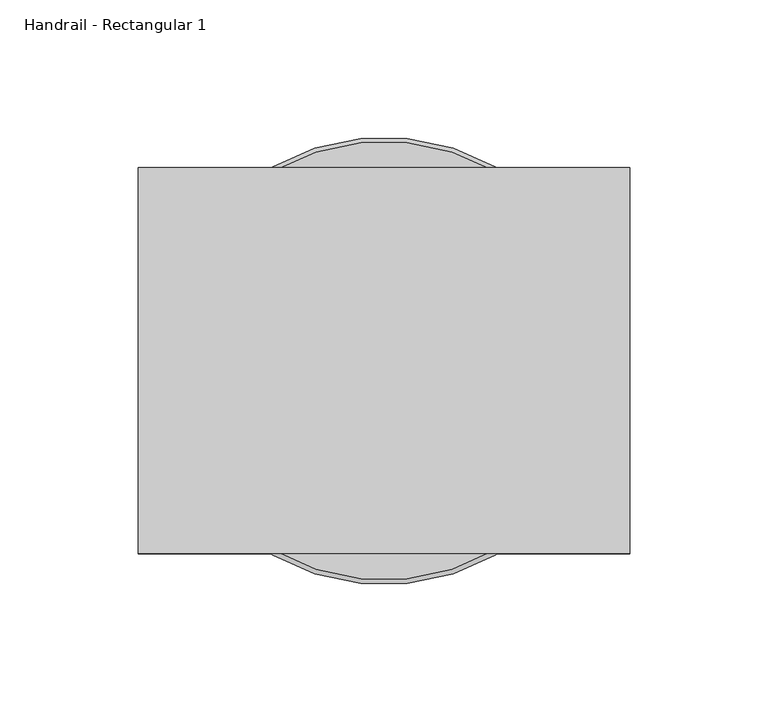
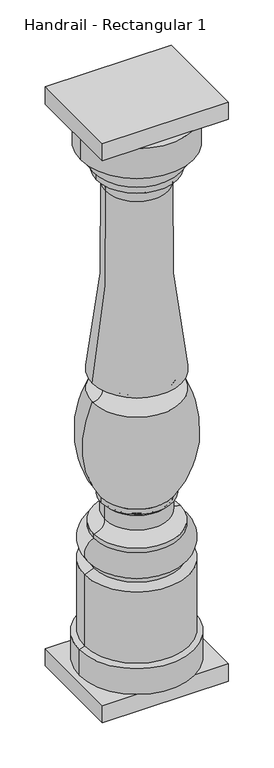
"""IFC4 building model written with IfcOpenShell, lengths in millimetres: railing geometry, Handrail - Rectangular 1."""

import ifcopenshell
import ifcopenshell.guid

model = None  # the IFC model being written
_history = None  # IfcOwnerHistory: only IFC2X3 demands one
_inside = {}  # id of a spatial element -> (the spatial element, [elements in it])
_under = {}  # id of a project, library or spatial element -> (it, [spatial elements below it])
_declared = {}  # id of a project -> (the project, [libraries it declares])
_typed = {}  # id of a type object -> (the type object, [elements of that type])
_made_of = {}  # id of a material, layer set ... -> (it, [elements and type objects made of it])


def new_model(schema):
    """Start an empty IFC model of exactly this schema.

    Asked for "IFC4X3", IfcOpenShell would pick the latest addendum, in which some entities
    have other attributes; the version numbers below select the first issue.
    IFC2X3 requires an IfcOwnerHistory on every rooted entity: one is made here for all.
    """
    global model, _history
    if schema == "IFC4X3":
        model = ifcopenshell.file(schema_version=(4, 3, 0, 0))
    else:
        model = ifcopenshell.file(schema=schema)
    _inside.clear()
    _under.clear()
    _declared.clear()
    _typed.clear()
    _made_of.clear()
    _history = None
    if model.schema == "IFC2X3":
        org = make("IfcOrganization", Name="unknown")
        user = make(
            "IfcPersonAndOrganization",
            ThePerson=make("IfcPerson", FamilyName="unknown"),
            TheOrganization=org,
        )
        app = make(
            "IfcApplication",
            ApplicationDeveloper=org,
            Version="unknown",
            ApplicationFullName="unknown",
            ApplicationIdentifier="unknown",
        )
        _history = make(
            "IfcOwnerHistory",
            OwningUser=user,
            OwningApplication=app,
            ChangeAction="ADDED",
            CreationDate=0,
        )
    return model


def make(cls, **values):
    """One entity of the class cls with the attributes given. An attribute that is None is left unset."""
    return model.create_entity(
        cls, **{name: value for name, value in values.items() if value is not None}
    )


def rooted(cls, **values):
    """An entity with a GlobalId (a new one), such as an element, a storey or a relation."""
    return make(cls, GlobalId=ifcopenshell.guid.new(), OwnerHistory=_history, **values)


def si_unit(unit_type, name, prefix=None):
    """IfcSIUnit, for example si_unit("LENGTHUNIT", "METRE", prefix="MILLI")."""
    return make("IfcSIUnit", UnitType=unit_type, Prefix=prefix, Name=name)


def assignment(units):
    """IfcUnitAssignment: the units of a project."""
    return None if units is None else make("IfcUnitAssignment", Units=units)


def point(xyz):
    """IfcCartesianPoint."""
    return None if xyz is None else make("IfcCartesianPoint", Coordinates=xyz)


def direction(xyz):
    """IfcDirection."""
    return None if xyz is None else make("IfcDirection", DirectionRatios=xyz)


def frame(location, z_axis=None, x_axis=None):
    """IfcAxis2Placement3D, a coordinate frame: its origin and axes. An axis left out is left unset."""
    return make(
        "IfcAxis2Placement3D",
        Location=point(location),
        Axis=direction(z_axis),
        RefDirection=direction(x_axis),
    )


def origin():
    """The frame at (0, 0, 0) with its axes left unset."""
    return frame((0.0, 0.0, 0.0))


def place(relative_to, where):
    """IfcLocalPlacement: puts the frame where relative to a parent placement (None: the world)."""
    return make(
        "IfcLocalPlacement", PlacementRelTo=relative_to, RelativePlacement=where
    )


def context(
    kind, dimensions, precision=None, world=None, true_north=None, identifier=None
):
    """IfcGeometricRepresentationContext, for example the 3D "Model" context."""
    return make(
        "IfcGeometricRepresentationContext",
        ContextIdentifier=identifier,
        ContextType=kind,
        CoordinateSpaceDimension=dimensions,
        Precision=precision,
        WorldCoordinateSystem=world,
        TrueNorth=true_north,
    )


def project(units=None, contexts=None):
    """IfcProject with its units and contexts."""
    return rooted(
        "IfcProject",
        Name="project",
        RepresentationContexts=contexts,
        UnitsInContext=assignment(units),
    )


def spatial(cls, under=None, at=None, **own):
    """A site, building, storey or space (cls), placed at a placement, below another one or the project."""
    s = rooted(cls, ObjectPlacement=at, **own)
    if under is not None:
        _under.setdefault(under.id(), (under, []))[1].append(s)
    return s


def polyline(points):
    """IfcPolyline through the points."""
    return make("IfcPolyline", Points=[point(p) for p in points])


def circle_curve(where, radius):
    """IfcCircle in the frame where."""
    return make("IfcCircle", Position=where, Radius=radius)


def ellipse_curve(where, semi_axis1, semi_axis2):
    """IfcEllipse in the frame where."""
    return make(
        "IfcEllipse", Position=where, SemiAxis1=semi_axis1, SemiAxis2=semi_axis2
    )


def trimmed(basis, trim1, trim2, sense, master):
    """IfcTrimmedCurve: the piece of a basis curve between two trims."""
    return make(
        "IfcTrimmedCurve",
        BasisCurve=basis,
        Trim1=trim1,
        Trim2=trim2,
        SenseAgreement=sense,
        MasterRepresentation=master,
    )


def outline(outer, holes=None, kind="AREA"):
    """IfcArbitraryClosedProfileDef: a profile drawn as a closed curve; with holes, ...WithVoids."""
    if holes is None:
        return make("IfcArbitraryClosedProfileDef", ProfileType=kind, OuterCurve=outer)
    return make(
        "IfcArbitraryProfileDefWithVoids",
        ProfileType=kind,
        OuterCurve=outer,
        InnerCurves=holes,
    )


def extrude(swept, where, along, depth):
    """IfcExtrudedAreaSolid: the profile swept, set in the frame where, extruded along a direction by depth."""
    return make(
        "IfcExtrudedAreaSolid",
        SweptArea=swept,
        Position=where,
        ExtrudedDirection=direction(along),
        Depth=depth,
    )


def shape(context_of_items, identifier, shape_type, items):
    """IfcShapeRepresentation: the items that make up one representation, for example the "Body"."""
    return make(
        "IfcShapeRepresentation",
        ContextOfItems=context_of_items,
        RepresentationIdentifier=identifier,
        RepresentationType=shape_type,
        Items=items,
    )


def source(mapping_origin, context_of_items, identifier, shape_type, items):
    """IfcRepresentationMap: a shape defined once, which mapped items show again and again."""
    return make(
        "IfcRepresentationMap",
        MappingOrigin=mapping_origin,
        MappedRepresentation=shape(context_of_items, identifier, shape_type, items),
    )


def transform(
    local_origin,
    x_axis=None,
    y_axis=None,
    z_axis=None,
    scale=None,
    scale2=None,
    scale3=None,
    uniform=True,
):
    """IfcCartesianTransformationOperator3D, or its non-uniform kind. x_axis, y_axis, z_axis: its Axis1, 2, 3."""
    if uniform:
        return make(
            "IfcCartesianTransformationOperator3D",
            Axis1=direction(x_axis),
            Axis2=direction(y_axis),
            LocalOrigin=point(local_origin),
            Scale=scale,
            Axis3=direction(z_axis),
        )
    return make(
        "IfcCartesianTransformationOperator3DnonUniform",
        Axis1=direction(x_axis),
        Axis2=direction(y_axis),
        LocalOrigin=point(local_origin),
        Scale=scale,
        Axis3=direction(z_axis),
        Scale2=scale2,
        Scale3=scale3,
    )


def mapped(mapping_source, mapping_target):
    """IfcMappedItem: shows the shape of a source again, moved by a transform."""
    return make(
        "IfcMappedItem", MappingSource=mapping_source, MappingTarget=mapping_target
    )


def made_of(thing, what):
    """Note that an element or type object is made of a material, layer set ...; save() writes the relation."""
    if what is not None:
        _made_of.setdefault(what.id(), (what, []))[1].append(thing)
    return thing


def element(
    cls,
    number,
    at=None,
    inside=None,
    cuts=None,
    type_object=None,
    material=None,
    context=None,
    identifier="Body",
    shape_type=None,
    held_by="IfcProductDefinitionShape",
    body=None,
    shapes=None,
    **own,
):
    """One element of the class cls, such as IfcWall. Its Tag is "e" and its number.

    at: its placement. inside: the storey or other place that contains it. cuts: it is an
    opening in that element (IfcRelVoidsElement). A single representation is given by context,
    identifier, shape_type and body (its items); several are given by shapes. held_by: the class
    of the entity that holds the representations. save() writes the other relations.
    """
    e = rooted(cls, Tag="e%d" % number, ObjectPlacement=at, **own)
    if body is not None:
        shapes = [shape(context, identifier, shape_type, body)]
    if shapes is not None:
        e.Representation = make(held_by, Representations=shapes)
    if inside is not None:
        _inside.setdefault(inside.id(), (inside, []))[1].append(e)
    if cuts is not None:
        rooted(
            "IfcRelVoidsElement", RelatingBuildingElement=cuts, RelatedOpeningElement=e
        )
    if type_object is not None:
        _typed.setdefault(type_object.id(), (type_object, []))[1].append(e)
    return made_of(e, material)


def aggregate(whole, parts):
    """IfcRelAggregates: a whole, such as a stair, and the parts it consists of."""
    return rooted("IfcRelAggregates", RelatingObject=whole, RelatedObjects=parts)


def save(model, path):
    """Write the relations noted so far, then the file.

    IfcRelAggregates (storeys below a building ...), IfcRelContainedInSpatialStructure (elements
    in a storey), IfcRelDefinesByType, IfcRelAssociatesMaterial and IfcRelDeclares: one each for
    every whole, place, type object, material and project.
    """
    for whole, parts in _under.values():
        aggregate(whole, parts)
    for where, things in _inside.values():
        rooted(
            "IfcRelContainedInSpatialStructure",
            RelatedElements=things,
            RelatingStructure=where,
        )
    for kind, things in _typed.values():
        rooted("IfcRelDefinesByType", RelatedObjects=things, RelatingType=kind)
    for what, things in _made_of.values():
        rooted("IfcRelAssociatesMaterial", RelatedObjects=things, RelatingMaterial=what)
    for by, libraries in _declared.values():
        rooted("IfcRelDeclares", RelatingContext=by, RelatedDefinitions=libraries)
    model.write(path)


def plane_surface(at):
    """IfcPlane: the flat surface through the origin of the frame at, square to its z axis."""
    return make("IfcPlane", Position=at)


def cylinder_surface(at, radius):
    """IfcCylindricalSurface: all points at the distance radius from the z axis of the frame at."""
    return make("IfcCylindricalSurface", Position=at, Radius=radius)


def revolved_surface(curve, axis_point, axis_direction):
    """IfcSurfaceOfRevolution: the curve turned about the line through axis_point along axis_direction."""
    return make(
        "IfcSurfaceOfRevolution",
        SweptCurve=make("IfcArbitraryOpenProfileDef", ProfileType="CURVE", Curve=curve),
        AxisPosition=make("IfcAxis1Placement", Location=point(axis_point), Axis=direction(axis_direction)),
    )


def advanced_brep(points, edges, surfaces, faces):
    """IfcAdvancedBrep: a solid bounded by faces that lie on surfaces and meet in shared edges.

    An edge is (start, end): straight between two places in points (the first is 0);
    or (start, end, curve); or (start, end, curve, False) where it runs against its curve.
    A face is (place in surfaces, loops), or (place, loops, False) where it looks against
    its surface's normal. A loop lists edges by number (the first is 1), with a minus sign
    where the edge is run from its end to its start. The first loop is the outer one.
    """
    corners = [point(p) for p in points]
    vertices = [make("IfcVertexPoint", VertexGeometry=c) for c in corners]
    made = []
    for start, end, *more in edges:
        made.append(
            make(
                "IfcEdgeCurve",
                EdgeStart=vertices[start],
                EdgeEnd=vertices[end],
                EdgeGeometry=more[0] if more else make("IfcPolyline", Points=[corners[start], corners[end]]),
                SameSense=more[1] if len(more) > 1 else True,
            )
        )
    hull = []
    for where, loops, *sense in faces:
        bounds = []
        for j, loop in enumerate(loops):
            ring = [make("IfcOrientedEdge", EdgeElement=made[abs(k) - 1], Orientation=k > 0) for k in loop]
            bounds.append(
                make(
                    "IfcFaceOuterBound" if j == 0 else "IfcFaceBound",
                    Bound=make("IfcEdgeLoop", EdgeList=ring),
                    Orientation=True,
                )
            )
        hull.append(make("IfcAdvancedFace", Bounds=bounds, FaceSurface=surfaces[where], SameSense=sense[0] if sense else True))
    return make("IfcAdvancedBrep", Outer=make("IfcClosedShell", CfsFaces=hull))


def handrail_rectangular_1_85a9581f(model_context):
    return source(origin(), model_context, "Body", "SolidModel", [
        advanced_brep(
        [(6614.0521895, -1665.6164768, 939.8), (6534.6771895, -1665.6164768, 939.8), (6693.4271895, -1665.6164768, 939.8), (6695.0146895, -1665.6164768, 127.0), (6533.0896895, -1665.6164768, 127.0), (6614.0521895, -1665.6164768, 127.0), (6695.0146895, -1665.6164768, 165.2785542), (6533.0896895, -1665.6164768, 165.2785542), (6687.8709395, -1665.6164768, 168.275), (6540.2334395, -1665.6164768, 168.275), (6687.8709395, -1665.6164768, 274.7335284), (6540.2334395, -1665.6164768, 274.7335284), (6675.1709395, -1665.6164768, 280.19375), (6552.9334395, -1665.6164768, 280.19375), (6675.1709395, -1665.6164768, 286.54375), (6552.9334395, -1665.6164768, 286.54375), (6675.1709395, -1665.6164768, 324.64375), (6552.9334395, -1665.6164768, 324.64375), (6675.1709395, -1665.6164768, 330.99375), (6552.9334395, -1665.6164768, 330.99375), (6659.4640435, -1665.6164768, 347.276159), (6568.6403356, -1665.6164768, 347.276159), (6659.4640435, -1665.6164768, 368.8906259), (6568.6403356, -1665.6164768, 368.8906259), (6664.0584395, -1665.6164768, 373.85625), (6564.0459395, -1665.6164768, 373.85625), (6664.0584395, -1665.6164768, 381.4842759), (6564.0459395, -1665.6164768, 381.4842759), (6676.7584395, -1665.6164768, 527.84375), (6551.3459395, -1665.6164768, 527.84375), (6676.7584395, -1665.6164768, 556.41875), (6551.3459395, -1665.6164768, 556.41875), (6658.2243377, -1665.6164768, 836.1713606), (6569.8800414, -1665.6164768, 836.1713606), (6671.2021895, -1665.6164768, 858.04375), (6556.9021895, -1665.6164768, 858.04375), (6671.2021895, -1665.6164768, 866.775), (6556.9021895, -1665.6164768, 866.775), (6682.3146895, -1665.6164768, 892.175), (6545.7896895, -1665.6164768, 892.175), (6693.4271895, -1665.6164768, 895.35), (6534.6771895, -1665.6164768, 895.35)],
        [
            (0, 1),
            (1, 2, circle_curve(frame((6614.0521895, -1665.6164768, 939.8), z_axis=(0.0, 0.0, 1.0), x_axis=(-1.0, 0.0, 0.0)), 79.375)),
            (2, 0),
            (2, 1, circle_curve(frame((6614.0521895, -1665.6164768, 939.8), z_axis=(0.0, 0.0, 1.0), x_axis=(-1.0, 0.0, 0.0)), 79.375)),
            (3, 4, circle_curve(frame((6614.0521895, -1665.6164768, 127.0), z_axis=(0.0, 0.0, -1.0), x_axis=(-1.0, 0.0, 0.0)), 80.9625)),
            (4, 5),
            (5, 3),
            (4, 3, circle_curve(frame((6614.0521895, -1665.6164768, 127.0), z_axis=(0.0, 0.0, -1.0), x_axis=(-1.0, 0.0, 0.0)), 80.9625)),
            (6, 7, circle_curve(frame((6614.0521895, -1665.6164768, 165.2785542), z_axis=(0.0, 0.0, -1.0), x_axis=(-1.0, 0.0, 0.0)), 80.9625)),
            (7, 4),
            (3, 6),
            (7, 6, circle_curve(frame((6614.0521895, -1665.6164768, 165.2785542), z_axis=(0.0, 0.0, -1.0), x_axis=(-1.0, 0.0, 0.0)), 80.9625)),
            (8, 9, circle_curve(frame((6614.0521895, -1665.6164768, 168.275), z_axis=(0.0, 0.0, -1.0), x_axis=(-1.0, 0.0, 0.0)), 73.81875)),
            (9, 7),
            (6, 8),
            (9, 8, circle_curve(frame((6614.0521895, -1665.6164768, 168.275), z_axis=(0.0, 0.0, -1.0), x_axis=(-1.0, 0.0, 0.0)), 73.81875)),
            (10, 11, circle_curve(frame((6614.0521895, -1665.6164768, 274.7335284), z_axis=(0.0, 0.0, -1.0), x_axis=(-1.0, 0.0, 0.0)), 73.81875)),
            (11, 9),
            (8, 10),
            (11, 10, circle_curve(frame((6614.0521895, -1665.6164768, 274.7335284), z_axis=(0.0, 0.0, -1.0), x_axis=(-1.0, 0.0, 0.0)), 73.81875)),
            (12, 13, circle_curve(frame((6614.0521895, -1665.6164768, 280.19375), z_axis=(0.0, 0.0, -1.0), x_axis=(-1.0, 0.0, 0.0)), 61.11875)),
            (13, 11),
            (10, 12),
            (13, 12, circle_curve(frame((6614.0521895, -1665.6164768, 280.19375), z_axis=(0.0, 0.0, -1.0), x_axis=(-1.0, 0.0, 0.0)), 61.11875)),
            (14, 15, circle_curve(frame((6614.0521895, -1665.6164768, 286.54375), z_axis=(0.0, 0.0, -1.0), x_axis=(-1.0, 0.0, 0.0)), 61.11875)),
            (15, 13),
            (12, 14),
            (15, 14, circle_curve(frame((6614.0521895, -1665.6164768, 286.54375), z_axis=(0.0, 0.0, -1.0), x_axis=(-1.0, 0.0, 0.0)), 61.11875)),
            (16, 17, circle_curve(frame((6614.0521895, -1665.6164768, 324.64375), z_axis=(0.0, 0.0, -1.0), x_axis=(-1.0, 0.0, 0.0)), 61.11875)),
            (17, 15, circle_curve(frame((6561.1987498, -1665.6164768, 305.59375), z_axis=(0.0, -1.0, 0.0), x_axis=(1.0, 0.0, 0.0)), 20.7657856)),
            (14, 16, circle_curve(frame((6666.9056293, -1665.6164768, 305.59375), z_axis=(0.0, -1.0, 0.0), x_axis=(-1.0, 0.0, 0.0)), 20.7657856)),
            (17, 16, circle_curve(frame((6614.0521895, -1665.6164768, 324.64375), z_axis=(0.0, 0.0, -1.0), x_axis=(-1.0, 0.0, 0.0)), 61.11875)),
            (18, 19, circle_curve(frame((6614.0521895, -1665.6164768, 330.99375), z_axis=(0.0, 0.0, -1.0), x_axis=(-1.0, 0.0, 0.0)), 61.11875)),
            (19, 17),
            (16, 18),
            (19, 18, circle_curve(frame((6614.0521895, -1665.6164768, 330.99375), z_axis=(0.0, 0.0, -1.0), x_axis=(-1.0, 0.0, 0.0)), 61.11875)),
            (20, 21, circle_curve(frame((6614.0521895, -1665.6164768, 347.276159), z_axis=(0.0, 0.0, -1.0), x_axis=(-1.0, 0.0, 0.0)), 45.4118539)),
            (21, 19, circle_curve(frame((6553.4004121, -1665.6164768, 346.26035), z_axis=(0.0, 1.0, 0.0), x_axis=(1.0, 0.0, 0.0)), 15.2737402)),
            (18, 20, circle_curve(frame((6674.703967, -1665.6164768, 346.26035), z_axis=(0.0, 1.0, 0.0), x_axis=(-1.0, 0.0, 0.0)), 15.2737402)),
            (21, 20, circle_curve(frame((6614.0521895, -1665.6164768, 347.276159), z_axis=(0.0, 0.0, -1.0), x_axis=(-1.0, 0.0, 0.0)), 45.4118539)),
            (22, 23, circle_curve(frame((6614.0521895, -1665.6164768, 368.8906259), z_axis=(0.0, 0.0, -1.0), x_axis=(-1.0, 0.0, 0.0)), 45.4118539)),
            (23, 21),
            (20, 22),
            (23, 22, circle_curve(frame((6614.0521895, -1665.6164768, 368.8906259), z_axis=(0.0, 0.0, -1.0), x_axis=(-1.0, 0.0, 0.0)), 45.4118539)),
            (24, 25, circle_curve(frame((6614.0521895, -1665.6164768, 373.85625), z_axis=(0.0, 0.0, -1.0), x_axis=(-1.0, 0.0, 0.0)), 50.00625)),
            (25, 23, circle_curve(frame((6563.7940931, -1665.6164768, 369.014959), z_axis=(0.0, 1.0, 0.0), x_axis=(1.0, 0.0, 0.0)), 4.8478372)),
            (22, 24, circle_curve(frame((6664.310286, -1665.6164768, 369.014959), z_axis=(0.0, 1.0, 0.0), x_axis=(-1.0, 0.0, 0.0)), 4.8478372)),
            (25, 24, circle_curve(frame((6614.0521895, -1665.6164768, 373.85625), z_axis=(0.0, 0.0, -1.0), x_axis=(-1.0, 0.0, 0.0)), 50.00625)),
            (26, 27, circle_curve(frame((6614.0521895, -1665.6164768, 381.4842759), z_axis=(0.0, 0.0, -1.0), x_axis=(-1.0, 0.0, 0.0)), 50.00625)),
            (27, 25),
            (24, 26),
            (27, 26, circle_curve(frame((6614.0521895, -1665.6164768, 381.4842759), z_axis=(0.0, 0.0, -1.0), x_axis=(-1.0, 0.0, 0.0)), 50.00625)),
            (28, 29, circle_curve(frame((6614.0521895, -1665.6164768, 527.84375), z_axis=(0.0, 0.0, -1.0), x_axis=(-1.0, 0.0, 0.0)), 62.70625)),
            (29, 27, circle_curve(frame((6681.6829206, -1665.6164768, 465.4226923), z_axis=(0.0, -1.0, 0.0), x_axis=(1.0, 0.0, 0.0)), 144.5133802)),
            (26, 28, circle_curve(frame((6546.4214585, -1665.6164768, 465.4226923), z_axis=(0.0, -1.0, 0.0), x_axis=(-1.0, 0.0, 0.0)), 144.5133802)),
            (29, 28, circle_curve(frame((6614.0521895, -1665.6164768, 527.84375), z_axis=(0.0, 0.0, -1.0), x_axis=(-1.0, 0.0, 0.0)), 62.70625)),
            (30, 31, circle_curve(frame((6614.0521895, -1665.6164768, 556.41875), z_axis=(0.0, 0.0, -1.0), x_axis=(-1.0, 0.0, 0.0)), 62.70625)),
            (31, 29, circle_curve(frame((6552.1940628, -1665.6164768, 542.13125), z_axis=(0.0, 1.0, 0.0), x_axis=(1.0, 0.0, 0.0)), 14.3126507)),
            (28, 30, circle_curve(frame((6675.9103163, -1665.6164768, 542.13125), z_axis=(0.0, 1.0, 0.0), x_axis=(-1.0, 0.0, 0.0)), 14.3126507)),
            (31, 30, circle_curve(frame((6614.0521895, -1665.6164768, 556.41875), z_axis=(0.0, 0.0, -1.0), x_axis=(-1.0, 0.0, 0.0)), 62.70625)),
            (32, 33, circle_curve(frame((6614.0521895, -1665.6164768, 836.1713606), z_axis=(0.0, 0.0, -1.0), x_axis=(-1.0, 0.0, 0.0)), 44.1721482)),
            (33, 31, circle_curve(frame((5440.060691, -1665.6164768, 770.5336134), z_axis=(0.0, 1.0, 0.0), x_axis=(1.0, 0.0, 0.0)), 1131.7243827)),
            (30, 32, circle_curve(frame((7788.0436881, -1665.6164768, 770.5336134), z_axis=(0.0, 1.0, 0.0), x_axis=(-1.0, 0.0, 0.0)), 1131.7243827)),
            (33, 32, circle_curve(frame((6614.0521895, -1665.6164768, 836.1713606), z_axis=(0.0, 0.0, -1.0), x_axis=(-1.0, 0.0, 0.0)), 44.1721482)),
            (34, 35, circle_curve(frame((6614.0521895, -1665.6164768, 858.04375), z_axis=(0.0, 0.0, -1.0), x_axis=(-1.0, 0.0, 0.0)), 57.15)),
            (35, 33, circle_curve(frame((6548.8577367, -1665.6164768, 838.4842616), z_axis=(0.0, 1.0, 0.0), x_axis=(1.0, 0.0, 0.0)), 21.1491562)),
            (32, 34, circle_curve(frame((6679.2466424, -1665.6164768, 838.4842616), z_axis=(0.0, 1.0, 0.0), x_axis=(-1.0, 0.0, 0.0)), 21.1491562)),
            (35, 34, circle_curve(frame((6614.0521895, -1665.6164768, 858.04375), z_axis=(0.0, 0.0, -1.0), x_axis=(-1.0, 0.0, 0.0)), 57.15)),
            (36, 37, circle_curve(frame((6614.0521895, -1665.6164768, 866.775), z_axis=(0.0, 0.0, -1.0), x_axis=(-1.0, 0.0, 0.0)), 57.15)),
            (37, 35),
            (34, 36),
            (37, 36, circle_curve(frame((6614.0521895, -1665.6164768, 866.775), z_axis=(0.0, 0.0, -1.0), x_axis=(-1.0, 0.0, 0.0)), 57.15)),
            (38, 39, circle_curve(frame((6614.0521895, -1665.6164768, 892.175), z_axis=(0.0, 0.0, -1.0), x_axis=(-1.0, 0.0, 0.0)), 68.2625)),
            (39, 37, circle_curve(frame((6575.1272944, -1665.6164768, 889.8793427), z_axis=(0.0, -1.0, 0.0), x_axis=(1.0, 0.0, 0.0)), 29.4272849)),
            (36, 38, circle_curve(frame((6652.9770847, -1665.6164768, 889.8793427), z_axis=(0.0, -1.0, 0.0), x_axis=(-1.0, 0.0, 0.0)), 29.4272849)),
            (39, 38, circle_curve(frame((6614.0521895, -1665.6164768, 892.175), z_axis=(0.0, 0.0, -1.0), x_axis=(-1.0, 0.0, 0.0)), 68.2625)),
            (40, 41, circle_curve(frame((6614.0521895, -1665.6164768, 895.35), z_axis=(0.0, 0.0, -1.0), x_axis=(-1.0, 0.0, 0.0)), 79.375)),
            (41, 39),
            (38, 40),
            (41, 40, circle_curve(frame((6614.0521895, -1665.6164768, 895.35), z_axis=(0.0, 0.0, -1.0), x_axis=(-1.0, 0.0, 0.0)), 79.375)),
            (1, 41),
            (40, 2),
        ],
        [
            plane_surface(frame((6614.0521895, -1665.6164768, 939.8), z_axis=(0.0, 0.0, 1.0), x_axis=(-1.0, 0.0, 0.0))),
            plane_surface(frame((6614.0521895, -1665.6164768, 127.0), z_axis=(0.0, 0.0, -1.0), x_axis=(-1.0, 0.0, 0.0))),
            cylinder_surface(frame((6614.0521895, -1665.6164768, 1009.65), z_axis=(0.0, 0.0, 1.0), x_axis=(-1.0, 0.0, 0.0)), 80.9625),
            revolved_surface(polyline([(6533.0896895, -1665.6164768, 165.2785542), (6540.2334395, -1665.6164768, 168.275)]), (6614.0521895, -1665.6164768, 1009.65), (0.0, 0.0, 1.0)),
            cylinder_surface(frame((6614.0521895, -1665.6164768, 1009.65), z_axis=(0.0, 0.0, 1.0), x_axis=(-1.0, 0.0, 0.0)), 73.81875),
            revolved_surface(polyline([(6540.2334395, -1665.6164768, 274.7335284), (6552.9334395, -1665.6164768, 280.19375)]), (6614.0521895, -1665.6164768, 1009.65), (0.0, 0.0, 1.0)),
            cylinder_surface(frame((6614.0521895, -1665.6164768, 1009.65), z_axis=(0.0, 0.0, 1.0), x_axis=(-1.0, 0.0, 0.0)), 61.11875),
            revolved_surface(trimmed(ellipse_curve(frame((6561.1987498, -1665.6164768, 305.59375), z_axis=(0.0, 1.0, 0.0), x_axis=(1.0, 0.0, 0.0)), 20.7657856, 20.7657856), [point((6552.9334395, -1665.6164768, 286.54375))], [point((6552.9334395, -1665.6164768, 324.64375))], True, "CARTESIAN"), (6614.0521895, -1665.6164768, 1009.65), (0.0, 0.0, 1.0)),
            revolved_surface(trimmed(ellipse_curve(frame((6553.4004121, -1665.6164768, 346.26035), z_axis=(0.0, -1.0, 0.0), x_axis=(1.0, 0.0, 0.0)), 15.2737402, 15.2737402), [point((6552.9334395, -1665.6164768, 330.99375))], [point((6568.6403356, -1665.6164768, 347.276159))], True, "CARTESIAN"), (6614.0521895, -1665.6164768, 1009.65), (0.0, 0.0, 1.0)),
            cylinder_surface(frame((6614.0521895, -1665.6164768, 1009.65), z_axis=(0.0, 0.0, 1.0), x_axis=(-1.0, 0.0, 0.0)), 45.4118539),
            revolved_surface(trimmed(ellipse_curve(frame((6563.7940931, -1665.6164768, 369.014959), z_axis=(0.0, -1.0, 0.0), x_axis=(1.0, 0.0, 0.0)), 4.8478372, 4.8478372), [point((6568.6403356, -1665.6164768, 368.8906259))], [point((6564.0459395, -1665.6164768, 373.85625))], True, "CARTESIAN"), (6614.0521895, -1665.6164768, 1009.65), (0.0, 0.0, 1.0)),
            cylinder_surface(frame((6614.0521895, -1665.6164768, 1009.65), z_axis=(0.0, 0.0, 1.0), x_axis=(-1.0, 0.0, 0.0)), 50.00625),
            revolved_surface(trimmed(ellipse_curve(frame((6681.6829206, -1665.6164768, 465.4226923), z_axis=(0.0, 1.0, 0.0), x_axis=(1.0, 0.0, 0.0)), 144.5133802, 144.5133802), [point((6564.0459395, -1665.6164768, 381.4842759))], [point((6551.3459395, -1665.6164768, 527.84375))], True, "CARTESIAN"), (6614.0521895, -1665.6164768, 1009.65), (0.0, 0.0, 1.0)),
            revolved_surface(trimmed(ellipse_curve(frame((6552.1940628, -1665.6164768, 542.13125), z_axis=(0.0, -1.0, 0.0), x_axis=(1.0, 0.0, 0.0)), 14.3126507, 14.3126507), [point((6551.3459395, -1665.6164768, 527.84375))], [point((6551.3459395, -1665.6164768, 556.41875))], True, "CARTESIAN"), (6614.0521895, -1665.6164768, 1009.65), (0.0, 0.0, 1.0)),
            revolved_surface(trimmed(ellipse_curve(frame((5440.060691, -1665.6164768, 770.5336134), z_axis=(0.0, -1.0, 0.0), x_axis=(1.0, 0.0, 0.0)), 1131.7243827, 1131.7243827), [point((6551.3459395, -1665.6164768, 556.41875))], [point((6569.8800414, -1665.6164768, 836.1713606))], True, "CARTESIAN"), (6614.0521895, -1665.6164768, 1009.65), (0.0, 0.0, 1.0)),
            revolved_surface(trimmed(ellipse_curve(frame((6548.8577367, -1665.6164768, 838.4842616), z_axis=(0.0, -1.0, 0.0), x_axis=(1.0, 0.0, 0.0)), 21.1491562, 21.1491562), [point((6569.8800414, -1665.6164768, 836.1713606))], [point((6556.9021895, -1665.6164768, 858.04375))], True, "CARTESIAN"), (6614.0521895, -1665.6164768, 1009.65), (0.0, 0.0, 1.0)),
            cylinder_surface(frame((6614.0521895, -1665.6164768, 1009.65), z_axis=(0.0, 0.0, 1.0), x_axis=(-1.0, 0.0, 0.0)), 57.15),
            revolved_surface(trimmed(ellipse_curve(frame((6575.1272944, -1665.6164768, 889.8793427), z_axis=(0.0, 1.0, 0.0), x_axis=(1.0, 0.0, 0.0)), 29.4272849, 29.4272849), [point((6556.9021895, -1665.6164768, 866.775))], [point((6545.7896895, -1665.6164768, 892.175))], True, "CARTESIAN"), (6614.0521895, -1665.6164768, 1009.65), (0.0, 0.0, 1.0)),
            revolved_surface(polyline([(6545.7896895, -1665.6164768, 892.175), (6534.6771895, -1665.6164768, 895.35)]), (6614.0521895, -1665.6164768, 1009.65), (0.0, 0.0, 1.0)),
            cylinder_surface(frame((6614.0521895, -1665.6164768, 1009.65), z_axis=(0.0, 0.0, 1.0), x_axis=(-1.0, 0.0, 0.0)), 79.375),
        ],
        [
            (0, [[1, 2, 3]]),
            (0, [[-3, 4, -1]]),
            (1, [[5, 6, 7]]),
            (1, [[8, -7, -6]]),
            (2, [[9, 10, -5, 11]]),
            (2, [[12, -11, -8, -10]]),
            (3, [[13, 14, -9, 15]]),
            (3, [[16, -15, -12, -14]]),
            (4, [[17, 18, -13, 19]]),
            (4, [[20, -19, -16, -18]]),
            (5, [[21, 22, -17, 23]]),
            (5, [[24, -23, -20, -22]]),
            (6, [[25, 26, -21, 27]]),
            (6, [[28, -27, -24, -26]]),
            (7, [[29, 30, -25, 31]]),
            (7, [[32, -31, -28, -30]]),
            (6, [[33, 34, -29, 35]]),
            (6, [[36, -35, -32, -34]]),
            (8, [[37, 38, -33, 39]]),
            (8, [[40, -39, -36, -38]]),
            (9, [[41, 42, -37, 43]]),
            (9, [[44, -43, -40, -42]]),
            (10, [[45, 46, -41, 47]]),
            (10, [[48, -47, -44, -46]]),
            (11, [[49, 50, -45, 51]]),
            (11, [[52, -51, -48, -50]]),
            (12, [[53, 54, -49, 55]]),
            (12, [[56, -55, -52, -54]]),
            (13, [[57, 58, -53, 59]]),
            (13, [[60, -59, -56, -58]]),
            (14, [[61, 62, -57, 63]]),
            (14, [[64, -63, -60, -62]]),
            (15, [[65, 66, -61, 67]]),
            (15, [[68, -67, -64, -66]]),
            (16, [[69, 70, -65, 71]]),
            (16, [[72, -71, -68, -70]]),
            (17, [[73, 74, -69, 75]]),
            (17, [[76, -75, -72, -74]]),
            (18, [[77, 78, -73, 79]]),
            (18, [[80, -79, -76, -78]]),
            (19, [[-2, 81, -77, 82]]),
            (19, [[-4, -82, -80, -81]]),
        ],
    ),
        extrude(outline(polyline([(6525.1521895, -1735.4664768), (6525.1521895, -1595.7664768), (6702.9521895, -1595.7664768), (6702.9521895, -1735.4664768), (6525.1521895, -1735.4664768)])), frame((0.0, 0.0, 101.6), z_axis=(0.0, 0.0, 1.0), x_axis=(1.0, 0.0, 0.0)), (0.0, 0.0, 1.0), 25.4),
        extrude(outline(polyline([(6525.1521895, -1595.7664768), (6702.9521895, -1595.7664768), (6702.9521895, -1735.4664768), (6525.1521895, -1735.4664768), (6525.1521895, -1595.7664768)])), frame((0.0, 0.0, 939.8), z_axis=(0.0, 0.0, 1.0), x_axis=(1.0, 0.0, 0.0)), (0.0, 0.0, 1.0), 25.4),
    ])


if __name__ == "__main__":
    model = new_model("IFC4")
    model_context = context("Model", 3, world=origin())
    ifc_project = project(units=[si_unit("LENGTHUNIT", "METRE", prefix="MILLI")], contexts=[model_context])
    site = spatial("IfcSite", under=ifc_project)
    building = spatial("IfcBuilding", under=site)
    placement = place(None, origin())
    handrail_rectangular_1_shape = handrail_rectangular_1_85a9581f(model_context)
    element("IfcRailing", 1, ObjectType="Handrail - Rectangular 1", at=placement, inside=building, context=model_context, shape_type="MappedRepresentation", body=[
        mapped(handrail_rectangular_1_shape, transform((0.0, 0.0, 0.0), x_axis=(1.0, 0.0, 0.0), y_axis=(0.0, 1.0, 0.0), z_axis=(0.0, 0.0, 1.0))),
    ])
    save(model, "model.ifc")
